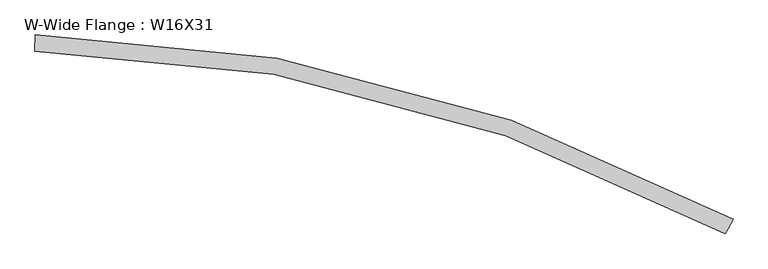
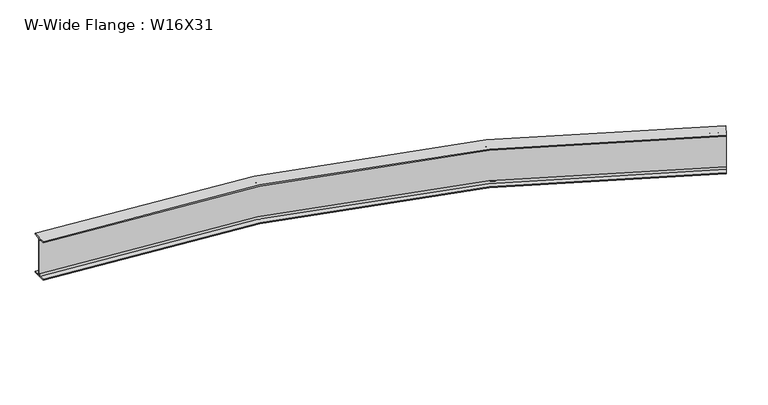
"""IFC4 building model written with IfcOpenShell, lengths in millimetres: beam geometry, W-Wide Flange : W16X31."""

from ifc_helpers import new_model, si_unit, point, frame, origin, place, context, project, spatial, polyline, circle_curve, ellipse_curve, trimmed, source, transform, mapped, element, save
from ifc_brep_helpers import plane_surface, cylinder_surface, revolved_surface, advanced_brep


def w_wide_flange_w16x31_2595adc3(model_context):
    return source(origin(), model_context, "Body", "AdvancedBrep", [
        advanced_brep(
        [(6106.6437094, -1493.8987471, -190.754), (6082.9245949, -1537.162934, -190.754), (6074.5603254, -1552.4195456, -173.355), (6074.5603254, -1552.4195456, 173.355), (6082.9245949, -1537.162934, 190.754), (6106.6437094, -1493.8987471, 190.754), (6106.6437094, -1493.8987471, 201.93), (6039.1190231, -1617.0652612, 201.93), (6039.1190231, -1617.0652612, 190.754), (6062.8381376, -1573.8010743, 190.754), (6071.202407, -1558.5444627, 173.355), (6071.202407, -1558.5444627, -173.355), (6062.8381376, -1573.8010743, -190.754), (6039.1190231, -1617.0652612, -190.754), (6039.1190231, -1617.0652612, -201.93), (6106.6437094, -1493.8987471, -201.93), (187.278858, 68.8503861, -190.754), (187.278858, 68.8503861, -201.93), (185.2080076, -71.5963477, -201.93), (185.2080076, -71.5963477, -190.754), (185.9354266, -22.2622102, -190.754), (186.1919424, -4.8651012, -173.355), (186.1919424, -4.8651012, 173.355), (185.9354266, -22.2622102, 190.754), (185.2080076, -71.5963477, 190.754), (185.2080076, -71.5963477, 201.93), (187.278858, 68.8503861, 201.93), (187.278858, 68.8503861, 190.754), (186.551439, 19.5162486, 190.754), (186.2949232, 2.1191396, 173.355), (186.2949232, 2.1191396, -173.355), (186.551439, 19.5162486, -190.754)],
        [
            (0, 1),
            (1, 2, circle_curve(frame((6082.9245949, -1537.162934, -173.355), z_axis=(-0.8768671529491877, 0.4807327699239839, 0.0), x_axis=(-0.4807327699239839, -0.8768671529491877, 0.0)), 17.399)),
            (2, 3),
            (3, 4, circle_curve(frame((6082.9245949, -1537.162934, 173.355), z_axis=(-0.8768671529491877, 0.4807327699239839, 0.0), x_axis=(-0.4807327699239839, -0.8768671529491877, 0.0)), 17.399)),
            (4, 5),
            (5, 6),
            (6, 7),
            (7, 8),
            (8, 9),
            (9, 10, circle_curve(frame((6062.8381376, -1573.8010743, 173.355), z_axis=(-0.8768671529491877, 0.4807327699239839, 0.0), x_axis=(-0.4807327699239839, -0.8768671529491877, 0.0)), 17.399)),
            (10, 11),
            (11, 12, circle_curve(frame((6062.8381376, -1573.8010743, -173.355), z_axis=(-0.8768671529491877, 0.4807327699239839, 0.0), x_axis=(-0.4807327699239839, -0.8768671529491877, 0.0)), 17.399)),
            (12, 13),
            (13, 14),
            (14, 15),
            (15, 0),
            (16, 17),
            (17, 18),
            (18, 19),
            (19, 20),
            (20, 21, circle_curve(frame((185.9354266, -22.2622102, -173.355), z_axis=(0.999891314050926, -0.014743136895265851, 0.0), x_axis=(-0.014743136895265851, -0.999891314050926, 0.0)), 17.399)),
            (21, 22),
            (22, 23, circle_curve(frame((185.9354266, -22.2622102, 173.355), z_axis=(0.999891314050926, -0.014743136895265851, 0.0), x_axis=(-0.014743136895265851, -0.999891314050926, 0.0)), 17.399)),
            (23, 24),
            (24, 25),
            (25, 26),
            (26, 27),
            (27, 28),
            (28, 29, circle_curve(frame((186.551439, 19.5162486, 173.355), z_axis=(0.999891314050926, -0.014743136895265851, 0.0), x_axis=(-0.014743136895265851, -0.999891314050926, 0.0)), 17.399)),
            (29, 30),
            (30, 31, circle_curve(frame((186.551439, 19.5162486, -173.355), z_axis=(0.999891314050926, -0.014743136895265851, 0.0), x_axis=(-0.014743136895265851, -0.999891314050926, 0.0)), 17.399)),
            (31, 16),
            (0, 16, circle_curve(frame((0.0, -12632.5512762, -190.754), z_axis=(0.0, 0.0, 1.0), x_axis=(-0.5014171979932397, -0.8652056365723748, 0.0)), 12702.7822762)),
            (31, 1, circle_curve(frame((0.0, -12632.5512762, -190.754), z_axis=(0.0, 0.0, -1.0), x_axis=(-0.5014171979932397, -0.8652056365723748, 0.0)), 12653.4427762)),
            (30, 2, circle_curve(frame((0.0, -12632.5512762, -173.355), z_axis=(0.0, 0.0, -1.0), x_axis=(-0.5014171979932397, -0.8652056365723748, 0.0)), 12636.0437762)),
            (29, 3, circle_curve(frame((0.0, -12632.5512762, 173.355), z_axis=(0.0, 0.0, -1.0), x_axis=(-0.5014171979932397, -0.8652056365723748, 0.0)), 12636.0437762)),
            (28, 4, circle_curve(frame((0.0, -12632.5512762, 190.754), z_axis=(0.0, 0.0, -1.0), x_axis=(-0.5014171979932397, -0.8652056365723748, 0.0)), 12653.4427762)),
            (27, 5, circle_curve(frame((0.0, -12632.5512762, 190.754), z_axis=(0.0, 0.0, -1.0), x_axis=(-0.5014171979932397, -0.8652056365723748, 0.0)), 12702.7822762)),
            (26, 6, circle_curve(frame((0.0, -12632.5512762, 201.93), z_axis=(0.0, 0.0, -1.0), x_axis=(-0.5014171979932397, -0.8652056365723748, 0.0)), 12702.7822762)),
            (25, 7, circle_curve(frame((0.0, -12632.5512762, 201.93), z_axis=(0.0, 0.0, -1.0), x_axis=(-0.5014171979932397, -0.8652056365723748, 0.0)), 12562.3202762)),
            (24, 8, circle_curve(frame((0.0, -12632.5512762, 190.754), z_axis=(0.0, 0.0, -1.0), x_axis=(-0.5014171979932397, -0.8652056365723748, 0.0)), 12562.3202762)),
            (23, 9, circle_curve(frame((0.0, -12632.5512762, 190.754), z_axis=(0.0, 0.0, -1.0), x_axis=(-0.5014171979932397, -0.8652056365723748, 0.0)), 12611.6597762)),
            (22, 10, circle_curve(frame((0.0, -12632.5512762, 173.355), z_axis=(0.0, 0.0, -1.0), x_axis=(-0.5014171979932397, -0.8652056365723748, 0.0)), 12629.0587762)),
            (21, 11, circle_curve(frame((0.0, -12632.5512762, -173.355), z_axis=(0.0, 0.0, -1.0), x_axis=(-0.5014171979932397, -0.8652056365723748, 0.0)), 12629.0587762)),
            (20, 12, circle_curve(frame((0.0, -12632.5512762, -190.754), z_axis=(0.0, 0.0, -1.0), x_axis=(-0.5014171979932397, -0.8652056365723748, 0.0)), 12611.6597762)),
            (19, 13, circle_curve(frame((0.0, -12632.5512762, -190.754), z_axis=(0.0, 0.0, -1.0), x_axis=(-0.5014171979932397, -0.8652056365723748, 0.0)), 12562.3202762)),
            (18, 14, circle_curve(frame((0.0, -12632.5512762, -201.93), z_axis=(0.0, 0.0, -1.0), x_axis=(-0.5014171979932397, -0.8652056365723748, 0.0)), 12562.3202762)),
            (17, 15, circle_curve(frame((0.0, -12632.5512762, -201.93), z_axis=(0.0, 0.0, -1.0), x_axis=(-0.5014171979932397, -0.8652056365723748, 0.0)), 12702.7822762)),
        ],
        [
            plane_surface(frame((6072.8813662, -1555.4820042, 0.0), z_axis=(0.8768671529491846, -0.4807327699239896, 0.0), x_axis=(0.0, 0.0, 1.0))),
            plane_surface(frame((186.2434328, -1.3729808, 0.0), z_axis=(-0.9998913140509259, 0.014743136895272237, 0.0), x_axis=(0.0, 0.0, 1.0))),
            plane_surface(frame((0.0, -12632.5512762, -190.754), z_axis=(0.0, 0.0, 1.0), x_axis=(-0.5014171979932397, -0.8652056365723748, 0.0))),
            revolved_surface(trimmed(ellipse_curve(frame((-6344.6538218, -23580.3812883, -173.355), z_axis=(-0.865205636572378, 0.5014171979932341, 0.0), x_axis=(0.5014171979932341, 0.865205636572378, 0.0)), 17.399, 17.399), [point((-6335.929664, -23565.3275754, -173.355))], [point((-6344.6538218, -23580.3812883, -190.754))], True, "CARTESIAN"), (0.0, -12632.5512762, 0.0), (0.0, 0.0, -1.0)),
            cylinder_surface(frame((0.0, -12632.5512762, 0.0), z_axis=(0.0, 0.0, -1.0), x_axis=(-0.5014171979932397, -0.8652056365723748, 0.0)), 12636.0437762),
            revolved_surface(trimmed(ellipse_curve(frame((-6344.6538218, -23580.3812883, 173.355), z_axis=(-0.865205636572378, 0.5014171979932341, 0.0), x_axis=(0.5014171979932341, 0.865205636572378, 0.0)), 17.399, 17.399), [point((-6344.6538218, -23580.3812883, 190.754))], [point((-6335.929664, -23565.3275754, 173.355))], True, "CARTESIAN"), (0.0, -12632.5512762, 0.0), (0.0, 0.0, -1.0)),
            plane_surface(frame((0.0, -12632.5512762, 190.754), z_axis=(0.0, 0.0, -1.0), x_axis=(-0.5014171979932397, -0.8652056365723748, 0.0))),
            cylinder_surface(frame((0.0, -12632.5512762, 0.0), z_axis=(0.0, 0.0, -1.0), x_axis=(-0.5014171979932397, -0.8652056365723748, 0.0)), 12702.7822762),
            plane_surface(frame((0.0, -12632.5512762, 201.93), z_axis=(0.0, 0.0, 1.0), x_axis=(-0.5014171979932397, -0.8652056365723748, 0.0))),
            revolved_surface(polyline([(-6298.963433185865, -23501.54158759567, 190.754), (-6298.963433185865, -23501.54158759567, 201.93)]), (0.0, -12632.5512762, 0.0), (0.0, 0.0, -1.0)),
            revolved_surface(trimmed(ellipse_curve(frame((-6323.703107, -23544.2304011, 173.355), z_axis=(-0.865205636572378, 0.5014171979932341, 0.0), x_axis=(0.5014171979932341, 0.865205636572378, 0.0)), 17.399, 17.399), [point((-6332.4272649, -23559.284114, 173.355))], [point((-6323.703107, -23544.2304011, 190.754))], True, "CARTESIAN"), (0.0, -12632.5512762, 0.0), (0.0, 0.0, -1.0)),
            revolved_surface(polyline([(-6332.427264854136, -23559.284113972055, -173.355), (-6332.427264854136, -23559.284113972055, 173.355)]), (0.0, -12632.5512762, 0.0), (0.0, 0.0, -1.0)),
            revolved_surface(trimmed(ellipse_curve(frame((-6323.703107, -23544.2304011, -173.355), z_axis=(-0.865205636572378, 0.5014171979932341, 0.0), x_axis=(0.5014171979932341, 0.865205636572378, 0.0)), 17.399, 17.399), [point((-6323.703107, -23544.2304011, -190.754))], [point((-6332.4272649, -23559.284114, -173.355))], True, "CARTESIAN"), (0.0, -12632.5512762, 0.0), (0.0, 0.0, -1.0)),
            revolved_surface(polyline([(-6298.963433185865, -23501.54158759567, -201.93), (-6298.963433185865, -23501.54158759567, -190.754)]), (0.0, -12632.5512762, 0.0), (0.0, 0.0, -1.0)),
            plane_surface(frame((0.0, -12632.5512762, -201.93), z_axis=(0.0, 0.0, -1.0), x_axis=(-0.5014171979932397, -0.8652056365723748, 0.0))),
        ],
        [
            (0, [[1, 2, 3, 4, 5, 6, 7, 8, 9, 10, 11, 12, 13, 14, 15, 16]]),
            (1, [[17, 18, 19, 20, 21, 22, 23, 24, 25, 26, 27, 28, 29, 30, 31, 32]]),
            (2, [[-1, 33, -32, 34]]),
            (3, [[-2, -34, -31, 35]]),
            (4, [[-3, -35, -30, 36]]),
            (5, [[-4, -36, -29, 37]]),
            (6, [[-5, -37, -28, 38]]),
            (7, [[-6, -38, -27, 39]]),
            (8, [[-7, -39, -26, 40]]),
            (9, [[-8, -40, -25, 41]]),
            (6, [[-9, -41, -24, 42]]),
            (10, [[-10, -42, -23, 43]]),
            (11, [[-11, -43, -22, 44]]),
            (12, [[-12, -44, -21, 45]]),
            (2, [[-13, -45, -20, 46]]),
            (13, [[-14, -46, -19, 47]]),
            (14, [[-15, -47, -18, 48]]),
            (7, [[-16, -48, -17, -33]]),
        ],
    ),
    ])


if __name__ == "__main__":
    model = new_model("IFC4")
    model_context = context("Model", 3, world=origin())
    ifc_project = project(units=[si_unit("LENGTHUNIT", "METRE", prefix="MILLI")], contexts=[model_context])
    site = spatial("IfcSite", under=ifc_project)
    building = spatial("IfcBuilding", under=site)
    placement = place(None, origin())
    w_wide_flange_w16x31_shape = w_wide_flange_w16x31_2595adc3(model_context)
    element("IfcBeam", 1, ObjectType="W-Wide Flange : W16X31", at=placement, inside=building, context=model_context, shape_type="MappedRepresentation", body=[
        mapped(w_wide_flange_w16x31_shape, transform((0.0, 0.0, 0.0), x_axis=(1.0, 0.0, 0.0), y_axis=(0.0, 1.0, 0.0), z_axis=(0.0, 0.0, 1.0))),
    ])
    save(model, "model.ifc")

# Revit data of these elements
# Type "W-Wide Flange : W16X31"
#   Assembly Code = "B10"
#   W = 31
#   Start Extension Calculation [instance default] = 10' - 0"
#   Start Extension [instance default] = -0' - 0 1/2"
#   End Extension Calculation [instance default] = 10' - 0"
#   End Extension [instance default] = -0' - 0 1/2"
#   Length [instance default] = 5' - 0"
#   bf = 0' - 5.53"
#   d = 1' - 3.9"
#   k = 0' - 1 1/8"
#   k2 = 0' - 0.685"
#   tf = 0' - 0.44"
#   tw = 0' - 0.275"
#   A = 0.0634028 SF
#   Beam Material [instance default] = Metal - Steel - ASTM A992
# Element 1 (IfcBeam, "W-Wide Flange : W16X31")
#   Materials on its faces: "Metal - Steel - ASTM A992"
# Materials
#   "Metal - Steel - ASTM A992": class "Metal", colour RGB 128 0 0, transparency 0
